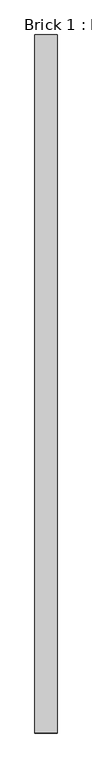
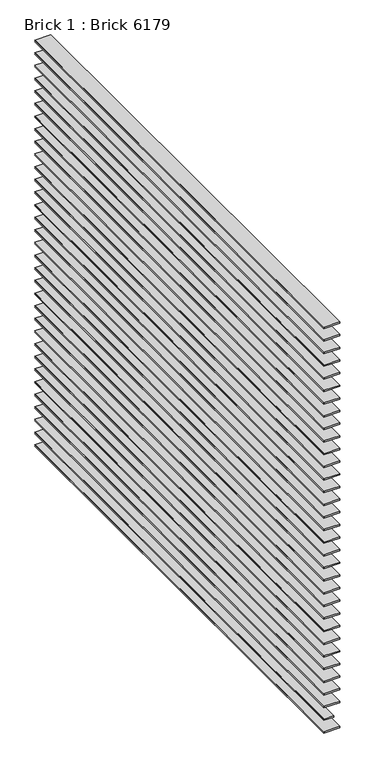
"""IFC4 building model written with IfcOpenShell, lengths in millimetres: proxy geometry, Brick 1 : Brick 6179."""

from ifc_helpers import new_model, si_unit, point, frame, frame_2d, origin, place, context, project, spatial, polyline, circle_curve, trimmed, segment, composite_curve, outline, extrude, source, transform, mapped, element, save


def brick_1_brick_6179_25ec3522(model_context):
    return source(origin(), model_context, "Body", "SweptSolid", [
        extrude(outline(composite_curve([segment(polyline([(37320.25, 10083.0612048), (37326.2029111, 10083.0612048), (37326.2029111, 10019.5612048)]), True, "CONTINUOUS"), segment(trimmed(circle_curve(frame_2d((37323.2264555, 10016.8521801)), 4.0246867), [point((37326.2029111, 10019.5612048))], [point((37320.25, 10019.5612048))], True, "CARTESIAN"), True, "CONTINUOUS"), segment(polyline([(37320.25, 10019.5612048), (37320.25, 10083.0612048)]), True, "CONTINUOUS")], self_intersect=False)), frame((0.0, 2217.3609988, 0.0), z_axis=(0.0, 1.0, 0.0), x_axis=(0.0, 0.0, 1.0)), (0.0, 0.0, 1.0), 2000.0),
        extrude(outline(composite_curve([segment(polyline([(37373.6875, 10059.8947267), (37379.6404111, 10059.8947267), (37379.6404111, 10019.5612048)]), True, "CONTINUOUS"), segment(trimmed(circle_curve(frame_2d((37376.6639555, 10016.8521801)), 4.0246867), [point((37379.6404111, 10019.5612048))], [point((37373.6875, 10019.5612048))], True, "CARTESIAN"), True, "CONTINUOUS"), segment(polyline([(37373.6875, 10019.5612048), (37373.6875, 10059.8947267)]), True, "CONTINUOUS")], self_intersect=False)), frame((0.0, 2217.3609988, 0.0), z_axis=(0.0, 1.0, 0.0), x_axis=(0.0, 0.0, 1.0)), (0.0, 0.0, 1.0), 2000.0),
        extrude(outline(composite_curve([segment(polyline([(37427.125, 10083.0612048), (37433.0779111, 10083.0612048), (37433.0779111, 10019.5612048)]), True, "CONTINUOUS"), segment(trimmed(circle_curve(frame_2d((37430.1014555, 10016.8521801)), 4.0246867), [point((37433.0779111, 10019.5612048))], [point((37427.125, 10019.5612048))], True, "CARTESIAN"), True, "CONTINUOUS"), segment(polyline([(37427.125, 10019.5612048), (37427.125, 10083.0612048)]), True, "CONTINUOUS")], self_intersect=False)), frame((0.0, 2217.3609988, 0.0), z_axis=(0.0, 1.0, 0.0), x_axis=(0.0, 0.0, 1.0)), (0.0, 0.0, 1.0), 2000.0),
        extrude(outline(composite_curve([segment(polyline([(37480.5625, 10083.0612048), (37486.5154111, 10083.0612048), (37486.5154111, 10019.5612048)]), True, "CONTINUOUS"), segment(trimmed(circle_curve(frame_2d((37483.5389555, 10016.8521801)), 4.0246867), [point((37486.5154111, 10019.5612048))], [point((37480.5625, 10019.5612048))], True, "CARTESIAN"), True, "CONTINUOUS"), segment(polyline([(37480.5625, 10019.5612048), (37480.5625, 10083.0612048)]), True, "CONTINUOUS")], self_intersect=False)), frame((0.0, 2217.3609988, 0.0), z_axis=(0.0, 1.0, 0.0), x_axis=(0.0, 0.0, 1.0)), (0.0, 0.0, 1.0), 2000.0),
        extrude(outline(composite_curve([segment(polyline([(37534.0, 10083.0612048), (37539.9529111, 10083.0612048), (37539.9529111, 10019.5612048)]), True, "CONTINUOUS"), segment(trimmed(circle_curve(frame_2d((37536.9764555, 10016.8521801)), 4.0246867), [point((37539.9529111, 10019.5612048))], [point((37534.0, 10019.5612048))], True, "CARTESIAN"), True, "CONTINUOUS"), segment(polyline([(37534.0, 10019.5612048), (37534.0, 10083.0612048)]), True, "CONTINUOUS")], self_intersect=False)), frame((0.0, 2217.3609988, 0.0), z_axis=(0.0, 1.0, 0.0), x_axis=(0.0, 0.0, 1.0)), (0.0, 0.0, 1.0), 2000.0),
        extrude(outline(composite_curve([segment(polyline([(37587.4375, 10083.0612048), (37593.3904111, 10083.0612048), (37593.3904111, 10019.5612048)]), True, "CONTINUOUS"), segment(trimmed(circle_curve(frame_2d((37590.4139555, 10016.8521801)), 4.0246867), [point((37593.3904111, 10019.5612048))], [point((37587.4375, 10019.5612048))], True, "CARTESIAN"), True, "CONTINUOUS"), segment(polyline([(37587.4375, 10019.5612048), (37587.4375, 10083.0612048)]), True, "CONTINUOUS")], self_intersect=False)), frame((0.0, 2217.3609988, 0.0), z_axis=(0.0, 1.0, 0.0), x_axis=(0.0, 0.0, 1.0)), (0.0, 0.0, 1.0), 2000.0),
        extrude(outline(composite_curve([segment(polyline([(37640.875, 10083.0612048), (37646.8279111, 10083.0612048), (37646.8279111, 10019.5612048)]), True, "CONTINUOUS"), segment(trimmed(circle_curve(frame_2d((37643.8514555, 10016.8521801)), 4.0246867), [point((37646.8279111, 10019.5612048))], [point((37640.875, 10019.5612048))], True, "CARTESIAN"), True, "CONTINUOUS"), segment(polyline([(37640.875, 10019.5612048), (37640.875, 10083.0612048)]), True, "CONTINUOUS")], self_intersect=False)), frame((0.0, 2217.3609988, 0.0), z_axis=(0.0, 1.0, 0.0), x_axis=(0.0, 0.0, 1.0)), (0.0, 0.0, 1.0), 2000.0),
        extrude(outline(composite_curve([segment(polyline([(37694.3125, 10083.0612048), (37700.2654111, 10083.0612048), (37700.2654111, 10019.5612048)]), True, "CONTINUOUS"), segment(trimmed(circle_curve(frame_2d((37697.2889555, 10016.8521801)), 4.0246867), [point((37700.2654111, 10019.5612048))], [point((37694.3125, 10019.5612048))], True, "CARTESIAN"), True, "CONTINUOUS"), segment(polyline([(37694.3125, 10019.5612048), (37694.3125, 10083.0612048)]), True, "CONTINUOUS")], self_intersect=False)), frame((0.0, 2217.3609988, 0.0), z_axis=(0.0, 1.0, 0.0), x_axis=(0.0, 0.0, 1.0)), (0.0, 0.0, 1.0), 2000.0),
        extrude(outline(composite_curve([segment(polyline([(37747.75, 10083.0612048), (37753.7029111, 10083.0612048), (37753.7029111, 10019.5612048)]), True, "CONTINUOUS"), segment(trimmed(circle_curve(frame_2d((37750.7264555, 10016.8521801)), 4.0246867), [point((37753.7029111, 10019.5612048))], [point((37747.75, 10019.5612048))], True, "CARTESIAN"), True, "CONTINUOUS"), segment(polyline([(37747.75, 10019.5612048), (37747.75, 10083.0612048)]), True, "CONTINUOUS")], self_intersect=False)), frame((0.0, 2217.3609988, 0.0), z_axis=(0.0, 1.0, 0.0), x_axis=(0.0, 0.0, 1.0)), (0.0, 0.0, 1.0), 2000.0),
        extrude(outline(composite_curve([segment(polyline([(37801.1875, 10083.0612048), (37807.1404111, 10083.0612048), (37807.1404111, 10019.5612048)]), True, "CONTINUOUS"), segment(trimmed(circle_curve(frame_2d((37804.1639555, 10016.8521801)), 4.0246867), [point((37807.1404111, 10019.5612048))], [point((37801.1875, 10019.5612048))], True, "CARTESIAN"), True, "CONTINUOUS"), segment(polyline([(37801.1875, 10019.5612048), (37801.1875, 10083.0612048)]), True, "CONTINUOUS")], self_intersect=False)), frame((0.0, 2217.3609988, 0.0), z_axis=(0.0, 1.0, 0.0), x_axis=(0.0, 0.0, 1.0)), (0.0, 0.0, 1.0), 2000.0),
        extrude(outline(composite_curve([segment(polyline([(37854.625, 10083.0612048), (37860.5779111, 10083.0612048), (37860.5779111, 10019.5612048)]), True, "CONTINUOUS"), segment(trimmed(circle_curve(frame_2d((37857.6014555, 10016.8521801)), 4.0246867), [point((37860.5779111, 10019.5612048))], [point((37854.625, 10019.5612048))], True, "CARTESIAN"), True, "CONTINUOUS"), segment(polyline([(37854.625, 10019.5612048), (37854.625, 10083.0612048)]), True, "CONTINUOUS")], self_intersect=False)), frame((0.0, 2217.3609988, 0.0), z_axis=(0.0, 1.0, 0.0), x_axis=(0.0, 0.0, 1.0)), (0.0, 0.0, 1.0), 2000.0),
        extrude(outline(composite_curve([segment(polyline([(37908.0625, 10083.0612048), (37914.0154111, 10083.0612048), (37914.0154111, 10019.5612048)]), True, "CONTINUOUS"), segment(trimmed(circle_curve(frame_2d((37911.0389555, 10016.8521801)), 4.0246867), [point((37914.0154111, 10019.5612048))], [point((37908.0625, 10019.5612048))], True, "CARTESIAN"), True, "CONTINUOUS"), segment(polyline([(37908.0625, 10019.5612048), (37908.0625, 10083.0612048)]), True, "CONTINUOUS")], self_intersect=False)), frame((0.0, 2217.3609988, 0.0), z_axis=(0.0, 1.0, 0.0), x_axis=(0.0, 0.0, 1.0)), (0.0, 0.0, 1.0), 2000.0),
        extrude(outline(composite_curve([segment(polyline([(37961.5, 10083.0612048), (37967.4529111, 10083.0612048), (37967.4529111, 10019.5612048)]), True, "CONTINUOUS"), segment(trimmed(circle_curve(frame_2d((37964.4764555, 10016.8521801)), 4.0246867), [point((37967.4529111, 10019.5612048))], [point((37961.5, 10019.5612048))], True, "CARTESIAN"), True, "CONTINUOUS"), segment(polyline([(37961.5, 10019.5612048), (37961.5, 10083.0612048)]), True, "CONTINUOUS")], self_intersect=False)), frame((0.0, 2217.3609988, 0.0), z_axis=(0.0, 1.0, 0.0), x_axis=(0.0, 0.0, 1.0)), (0.0, 0.0, 1.0), 2000.0),
        extrude(outline(composite_curve([segment(polyline([(38014.9375, 10083.0612048), (38020.8904111, 10083.0612048), (38020.8904111, 10019.5612048)]), True, "CONTINUOUS"), segment(trimmed(circle_curve(frame_2d((38017.9139555, 10016.8521801)), 4.0246867), [point((38020.8904111, 10019.5612048))], [point((38014.9375, 10019.5612048))], True, "CARTESIAN"), True, "CONTINUOUS"), segment(polyline([(38014.9375, 10019.5612048), (38014.9375, 10083.0612048)]), True, "CONTINUOUS")], self_intersect=False)), frame((0.0, 2217.3609988, 0.0), z_axis=(0.0, 1.0, 0.0), x_axis=(0.0, 0.0, 1.0)), (0.0, 0.0, 1.0), 2000.0),
        extrude(outline(composite_curve([segment(polyline([(38068.375, 10083.0612048), (38074.3279111, 10083.0612048), (38074.3279111, 10019.5612048)]), True, "CONTINUOUS"), segment(trimmed(circle_curve(frame_2d((38071.3514555, 10016.8521801)), 4.0246867), [point((38074.3279111, 10019.5612048))], [point((38068.375, 10019.5612048))], True, "CARTESIAN"), True, "CONTINUOUS"), segment(polyline([(38068.375, 10019.5612048), (38068.375, 10083.0612048)]), True, "CONTINUOUS")], self_intersect=False)), frame((0.0, 2217.3609988, 0.0), z_axis=(0.0, 1.0, 0.0), x_axis=(0.0, 0.0, 1.0)), (0.0, 0.0, 1.0), 2000.0),
        extrude(outline(composite_curve([segment(polyline([(38121.8125, 10083.0612048), (38127.7654111, 10083.0612048), (38127.7654111, 10019.5612048)]), True, "CONTINUOUS"), segment(trimmed(circle_curve(frame_2d((38124.7889555, 10016.8521801)), 4.0246867), [point((38127.7654111, 10019.5612048))], [point((38121.8125, 10019.5612048))], True, "CARTESIAN"), True, "CONTINUOUS"), segment(polyline([(38121.8125, 10019.5612048), (38121.8125, 10083.0612048)]), True, "CONTINUOUS")], self_intersect=False)), frame((0.0, 2217.3609988, 0.0), z_axis=(0.0, 1.0, 0.0), x_axis=(0.0, 0.0, 1.0)), (0.0, 0.0, 1.0), 2000.0),
        extrude(outline(composite_curve([segment(polyline([(38175.25, 10083.0612048), (38181.2029111, 10083.0612048), (38181.2029111, 10019.5612048)]), True, "CONTINUOUS"), segment(trimmed(circle_curve(frame_2d((38178.2264555, 10016.8521801)), 4.0246867), [point((38181.2029111, 10019.5612048))], [point((38175.25, 10019.5612048))], True, "CARTESIAN"), True, "CONTINUOUS"), segment(polyline([(38175.25, 10019.5612048), (38175.25, 10083.0612048)]), True, "CONTINUOUS")], self_intersect=False)), frame((0.0, 2217.3609988, 0.0), z_axis=(0.0, 1.0, 0.0), x_axis=(0.0, 0.0, 1.0)), (0.0, 0.0, 1.0), 2000.0),
        extrude(outline(composite_curve([segment(polyline([(38228.6875, 10083.0612048), (38234.6404111, 10083.0612048), (38234.6404111, 10019.5612048)]), True, "CONTINUOUS"), segment(trimmed(circle_curve(frame_2d((38231.6639555, 10016.8521801)), 4.0246867), [point((38234.6404111, 10019.5612048))], [point((38228.6875, 10019.5612048))], True, "CARTESIAN"), True, "CONTINUOUS"), segment(polyline([(38228.6875, 10019.5612048), (38228.6875, 10083.0612048)]), True, "CONTINUOUS")], self_intersect=False)), frame((0.0, 2217.3609988, 0.0), z_axis=(0.0, 1.0, 0.0), x_axis=(0.0, 0.0, 1.0)), (0.0, 0.0, 1.0), 2000.0),
        extrude(outline(composite_curve([segment(polyline([(38282.125, 10083.0612048), (38288.0779111, 10083.0612048), (38288.0779111, 10019.5612048)]), True, "CONTINUOUS"), segment(trimmed(circle_curve(frame_2d((38285.1014555, 10016.8521801)), 4.0246867), [point((38288.0779111, 10019.5612048))], [point((38282.125, 10019.5612048))], True, "CARTESIAN"), True, "CONTINUOUS"), segment(polyline([(38282.125, 10019.5612048), (38282.125, 10083.0612048)]), True, "CONTINUOUS")], self_intersect=False)), frame((0.0, 2217.3609988, 0.0), z_axis=(0.0, 1.0, 0.0), x_axis=(0.0, 0.0, 1.0)), (0.0, 0.0, 1.0), 2000.0),
        extrude(outline(composite_curve([segment(polyline([(38335.5625, 10083.0612048), (38341.5154111, 10083.0612048), (38341.5154111, 10019.5612048)]), True, "CONTINUOUS"), segment(trimmed(circle_curve(frame_2d((38338.5389555, 10016.8521801)), 4.0246867), [point((38341.5154111, 10019.5612048))], [point((38335.5625, 10019.5612048))], True, "CARTESIAN"), True, "CONTINUOUS"), segment(polyline([(38335.5625, 10019.5612048), (38335.5625, 10083.0612048)]), True, "CONTINUOUS")], self_intersect=False)), frame((0.0, 2217.3609988, 0.0), z_axis=(0.0, 1.0, 0.0), x_axis=(0.0, 0.0, 1.0)), (0.0, 0.0, 1.0), 2000.0),
        extrude(outline(composite_curve([segment(polyline([(38389.0, 10083.0612048), (38394.9529111, 10083.0612048), (38394.9529111, 10019.5612048)]), True, "CONTINUOUS"), segment(trimmed(circle_curve(frame_2d((38391.9764555, 10016.8521801)), 4.0246867), [point((38394.9529111, 10019.5612048))], [point((38389.0, 10019.5612048))], True, "CARTESIAN"), True, "CONTINUOUS"), segment(polyline([(38389.0, 10019.5612048), (38389.0, 10083.0612048)]), True, "CONTINUOUS")], self_intersect=False)), frame((0.0, 2217.3609988, 0.0), z_axis=(0.0, 1.0, 0.0), x_axis=(0.0, 0.0, 1.0)), (0.0, 0.0, 1.0), 2000.0),
        extrude(outline(composite_curve([segment(polyline([(38442.4375, 10083.0612048), (38448.3904111, 10083.0612048), (38448.3904111, 10019.5612048)]), True, "CONTINUOUS"), segment(trimmed(circle_curve(frame_2d((38445.4139555, 10016.8521801)), 4.0246867), [point((38448.3904111, 10019.5612048))], [point((38442.4375, 10019.5612048))], True, "CARTESIAN"), True, "CONTINUOUS"), segment(polyline([(38442.4375, 10019.5612048), (38442.4375, 10083.0612048)]), True, "CONTINUOUS")], self_intersect=False)), frame((0.0, 2217.3609988, 0.0), z_axis=(0.0, 1.0, 0.0), x_axis=(0.0, 0.0, 1.0)), (0.0, 0.0, 1.0), 2000.0),
        extrude(outline(composite_curve([segment(polyline([(38495.875, 10083.0612048), (38501.8279111, 10083.0612048), (38501.8279111, 10019.5612048)]), True, "CONTINUOUS"), segment(trimmed(circle_curve(frame_2d((38498.8514555, 10016.8521801)), 4.0246867), [point((38501.8279111, 10019.5612048))], [point((38495.875, 10019.5612048))], True, "CARTESIAN"), True, "CONTINUOUS"), segment(polyline([(38495.875, 10019.5612048), (38495.875, 10083.0612048)]), True, "CONTINUOUS")], self_intersect=False)), frame((0.0, 2217.3609988, 0.0), z_axis=(0.0, 1.0, 0.0), x_axis=(0.0, 0.0, 1.0)), (0.0, 0.0, 1.0), 2000.0),
        extrude(outline(composite_curve([segment(polyline([(38549.3125, 10083.0612048), (38555.2654111, 10083.0612048), (38555.2654111, 10019.5612048)]), True, "CONTINUOUS"), segment(trimmed(circle_curve(frame_2d((38552.2889555, 10016.8521801)), 4.0246867), [point((38555.2654111, 10019.5612048))], [point((38549.3125, 10019.5612048))], True, "CARTESIAN"), True, "CONTINUOUS"), segment(polyline([(38549.3125, 10019.5612048), (38549.3125, 10083.0612048)]), True, "CONTINUOUS")], self_intersect=False)), frame((0.0, 2217.3609988, 0.0), z_axis=(0.0, 1.0, 0.0), x_axis=(0.0, 0.0, 1.0)), (0.0, 0.0, 1.0), 2000.0),
        extrude(outline(composite_curve([segment(polyline([(38602.75, 10083.0612048), (38608.7029111, 10083.0612048), (38608.7029111, 10019.5612048)]), True, "CONTINUOUS"), segment(trimmed(circle_curve(frame_2d((38605.7264555, 10016.8521801)), 4.0246867), [point((38608.7029111, 10019.5612048))], [point((38602.75, 10019.5612048))], True, "CARTESIAN"), True, "CONTINUOUS"), segment(polyline([(38602.75, 10019.5612048), (38602.75, 10083.0612048)]), True, "CONTINUOUS")], self_intersect=False)), frame((0.0, 2217.3609988, 0.0), z_axis=(0.0, 1.0, 0.0), x_axis=(0.0, 0.0, 1.0)), (0.0, 0.0, 1.0), 2000.0),
        extrude(outline(composite_curve([segment(polyline([(38656.1875, 10083.0612048), (38662.1404111, 10083.0612048), (38662.1404111, 10019.5612048)]), True, "CONTINUOUS"), segment(trimmed(circle_curve(frame_2d((38659.1639555, 10016.8521801)), 4.0246867), [point((38662.1404111, 10019.5612048))], [point((38656.1875, 10019.5612048))], True, "CARTESIAN"), True, "CONTINUOUS"), segment(polyline([(38656.1875, 10019.5612048), (38656.1875, 10083.0612048)]), True, "CONTINUOUS")], self_intersect=False)), frame((0.0, 2217.3609988, 0.0), z_axis=(0.0, 1.0, 0.0), x_axis=(0.0, 0.0, 1.0)), (0.0, 0.0, 1.0), 2000.0),
        extrude(outline(composite_curve([segment(polyline([(38709.625, 10083.0612048), (38715.5779111, 10083.0612048), (38715.5779111, 10019.5612048)]), True, "CONTINUOUS"), segment(trimmed(circle_curve(frame_2d((38712.6014555, 10016.8521801)), 4.0246867), [point((38715.5779111, 10019.5612048))], [point((38709.625, 10019.5612048))], True, "CARTESIAN"), True, "CONTINUOUS"), segment(polyline([(38709.625, 10019.5612048), (38709.625, 10083.0612048)]), True, "CONTINUOUS")], self_intersect=False)), frame((0.0, 2217.3609988, 0.0), z_axis=(0.0, 1.0, 0.0), x_axis=(0.0, 0.0, 1.0)), (0.0, 0.0, 1.0), 2000.0),
        extrude(outline(composite_curve([segment(polyline([(38763.0625, 10083.0612048), (38769.0154111, 10083.0612048), (38769.0154111, 10019.5612048)]), True, "CONTINUOUS"), segment(trimmed(circle_curve(frame_2d((38766.0389555, 10016.8521801)), 4.0246867), [point((38769.0154111, 10019.5612048))], [point((38763.0625, 10019.5612048))], True, "CARTESIAN"), True, "CONTINUOUS"), segment(polyline([(38763.0625, 10019.5612048), (38763.0625, 10083.0612048)]), True, "CONTINUOUS")], self_intersect=False)), frame((0.0, 2217.3609988, 0.0), z_axis=(0.0, 1.0, 0.0), x_axis=(0.0, 0.0, 1.0)), (0.0, 0.0, 1.0), 2000.0),
        extrude(outline(composite_curve([segment(polyline([(38816.5, 10083.0612048), (38822.4529111, 10083.0612048), (38822.4529111, 10019.5612048)]), True, "CONTINUOUS"), segment(trimmed(circle_curve(frame_2d((38819.4764555, 10016.8521801)), 4.0246867), [point((38822.4529111, 10019.5612048))], [point((38816.5, 10019.5612048))], True, "CARTESIAN"), True, "CONTINUOUS"), segment(polyline([(38816.5, 10019.5612048), (38816.5, 10083.0612048)]), True, "CONTINUOUS")], self_intersect=False)), frame((0.0, 2217.3609988, 0.0), z_axis=(0.0, 1.0, 0.0), x_axis=(0.0, 0.0, 1.0)), (0.0, 0.0, 1.0), 2000.0),
        extrude(outline(composite_curve([segment(polyline([(38869.9375, 10083.0612048), (38875.8904111, 10083.0612048), (38875.8904111, 10019.5612048)]), True, "CONTINUOUS"), segment(trimmed(circle_curve(frame_2d((38872.9139555, 10016.8521801)), 4.0246867), [point((38875.8904111, 10019.5612048))], [point((38869.9375, 10019.5612048))], True, "CARTESIAN"), True, "CONTINUOUS"), segment(polyline([(38869.9375, 10019.5612048), (38869.9375, 10083.0612048)]), True, "CONTINUOUS")], self_intersect=False)), frame((0.0, 2217.3609988, 0.0), z_axis=(0.0, 1.0, 0.0), x_axis=(0.0, 0.0, 1.0)), (0.0, 0.0, 1.0), 2000.0),
        extrude(outline(composite_curve([segment(polyline([(38923.375, 10083.0612048), (38929.3279111, 10083.0612048), (38929.3279111, 10019.5612048)]), True, "CONTINUOUS"), segment(trimmed(circle_curve(frame_2d((38926.3514555, 10016.8521801)), 4.0246867), [point((38929.3279111, 10019.5612048))], [point((38923.375, 10019.5612048))], True, "CARTESIAN"), True, "CONTINUOUS"), segment(polyline([(38923.375, 10019.5612048), (38923.375, 10083.0612048)]), True, "CONTINUOUS")], self_intersect=False)), frame((0.0, 2217.3609988, 0.0), z_axis=(0.0, 1.0, 0.0), x_axis=(0.0, 0.0, 1.0)), (0.0, 0.0, 1.0), 2000.0),
        extrude(outline(composite_curve([segment(polyline([(38976.8125, 10083.0612048), (38982.7654111, 10083.0612048), (38982.7654111, 10019.5612048)]), True, "CONTINUOUS"), segment(trimmed(circle_curve(frame_2d((38979.7889555, 10016.8521801)), 4.0246867), [point((38982.7654111, 10019.5612048))], [point((38976.8125, 10019.5612048))], True, "CARTESIAN"), True, "CONTINUOUS"), segment(polyline([(38976.8125, 10019.5612048), (38976.8125, 10083.0612048)]), True, "CONTINUOUS")], self_intersect=False)), frame((0.0, 2217.3609988, 0.0), z_axis=(0.0, 1.0, 0.0), x_axis=(0.0, 0.0, 1.0)), (0.0, 0.0, 1.0), 2000.0),
        extrude(outline(composite_curve([segment(polyline([(39030.25, 10083.0612048), (39036.2029111, 10083.0612048), (39036.2029111, 10019.5612048)]), True, "CONTINUOUS"), segment(trimmed(circle_curve(frame_2d((39033.2264555, 10016.8521801)), 4.0246867), [point((39036.2029111, 10019.5612048))], [point((39030.25, 10019.5612048))], True, "CARTESIAN"), True, "CONTINUOUS"), segment(polyline([(39030.25, 10019.5612048), (39030.25, 10083.0612048)]), True, "CONTINUOUS")], self_intersect=False)), frame((0.0, 2217.3609988, 0.0), z_axis=(0.0, 1.0, 0.0), x_axis=(0.0, 0.0, 1.0)), (0.0, 0.0, 1.0), 2000.0),
    ])


if __name__ == "__main__":
    model = new_model("IFC4")
    model_context = context("Model", 3, world=origin())
    ifc_project = project(units=[si_unit("LENGTHUNIT", "METRE", prefix="MILLI")], contexts=[model_context])
    site = spatial("IfcSite", under=ifc_project)
    building = spatial("IfcBuilding", under=site)
    placement = place(None, origin())
    brick_1_brick_6179_shape = brick_1_brick_6179_25ec3522(model_context)
    element("IfcBuildingElementProxy", 1, Name="Brick 1 : Brick 6179", ObjectType="Brick 1 : Brick 6179", at=placement, inside=building, context=model_context, shape_type="MappedRepresentation", body=[
        mapped(brick_1_brick_6179_shape, transform((0.0, 0.0, 0.0), x_axis=(1.0, 0.0, 0.0), y_axis=(0.0, 1.0, 0.0), z_axis=(0.0, 0.0, 1.0))),
    ])
    save(model, "model.ifc")

# Revit data of these elements
# Type "Brick 1 : Brick 6179"
#   NameOverride = "Brick"
# Element 1 (IfcBuildingElementProxy, "Brick 1 : Brick 6179")
#   Materials on its faces: "MORTAR BED"
# Materials
#   "MORTAR BED": class "Unassigned", colour RGB 186 186 186, transparency 0, Cost = 0
